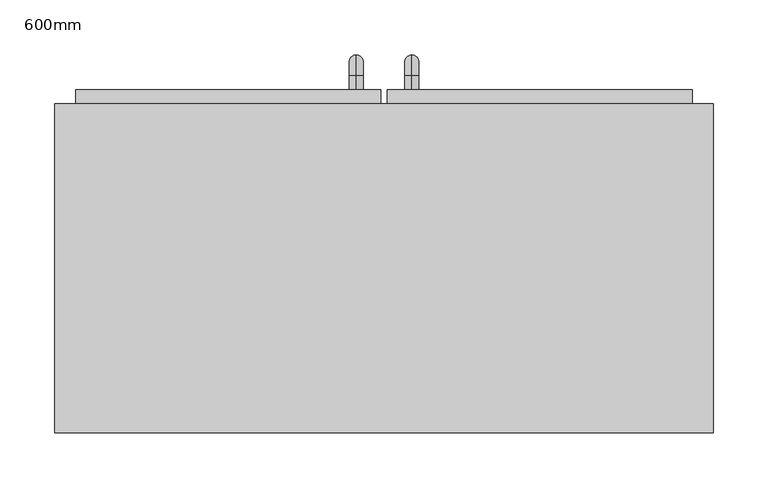
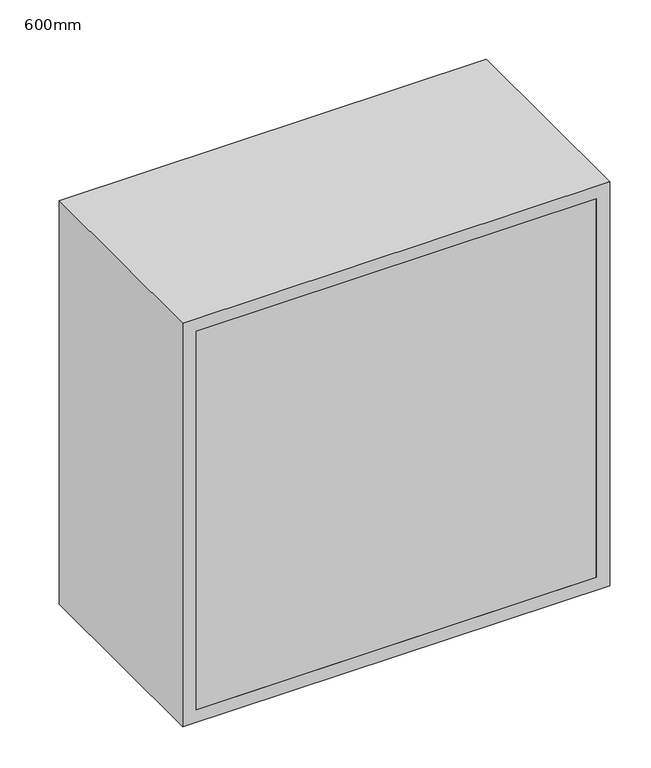
"""IFC4 building model written with IfcOpenShell, lengths in millimetres: furniture geometry, Armário superior-Porta dupla com vidro-Parede : 600mm."""

from ifc_helpers import new_model, si_unit, point, frame, origin, place, context, project, spatial, polyline, circle_curve, ellipse_curve, trimmed, outline, extrude, source, transform, mapped, element, save
from ifc_brep_helpers import plane_surface, cylinder_surface, revolved_surface, advanced_brep


def furniture_600mm_0b7ed25a(model_context):
    return source(origin(), model_context, "Body", "SolidModel", [
        advanced_brep(
        [(55.1711628, 412.7, 1546.05), (55.1711628, 412.7, 1558.75), (55.1711628, 425.4, 1546.05), (55.1711628, 425.4, 1558.75), (55.1711628, 444.45, 1539.7), (55.1711628, 431.75, 1539.7), (55.1711628, 431.75, 1463.5), (55.1711628, 444.45, 1463.5), (55.1711628, 425.4, 1444.45), (55.1711628, 425.4, 1457.15), (55.1711628, 412.7, 1457.15), (55.1711628, 412.7, 1444.45)],
        [
            (0, 1, circle_curve(frame((55.1711628, 412.7, 1552.4), z_axis=(0.0, -1.0, 0.0), x_axis=(0.0, 0.0, -1.0)), 6.35)),
            (1, 0, circle_curve(frame((55.1711628, 412.7, 1552.4), z_axis=(0.0, -1.0, 0.0), x_axis=(0.0, 0.0, -1.0)), 6.35)),
            (0, 2),
            (2, 3, circle_curve(frame((55.1711628, 425.4, 1552.4), z_axis=(0.0, -1.0, 0.0), x_axis=(0.0, 0.0, -1.0)), 6.35)),
            (3, 1),
            (3, 2, circle_curve(frame((55.1711628, 425.4, 1552.4), z_axis=(0.0, -1.0, 0.0), x_axis=(0.0, 0.0, -1.0)), 6.35)),
            (4, 3, circle_curve(frame((55.1711628, 425.4, 1539.7), z_axis=(1.0, 0.0, 0.0), x_axis=(0.0, 0.0, 1.0)), 19.05)),
            (2, 5, circle_curve(frame((55.1711628, 425.4, 1539.7), z_axis=(-1.0, 0.0, 0.0), x_axis=(0.0, 0.0, 1.0)), 6.35)),
            (5, 4, circle_curve(frame((55.1711628, 438.1, 1539.7), z_axis=(0.0, 0.0, 1.0), x_axis=(0.0, -1.0, 0.0)), 6.35)),
            (4, 5, circle_curve(frame((55.1711628, 438.1, 1539.7), z_axis=(0.0, 0.0, 1.0), x_axis=(0.0, -1.0, 0.0)), 6.35)),
            (5, 6),
            (6, 7, circle_curve(frame((55.1711628, 438.1, 1463.5), z_axis=(0.0, 0.0, 1.0), x_axis=(0.0, -1.0, 0.0)), 6.35)),
            (7, 4),
            (7, 6, circle_curve(frame((55.1711628, 438.1, 1463.5), z_axis=(0.0, 0.0, 1.0), x_axis=(0.0, -1.0, 0.0)), 6.35)),
            (8, 7, circle_curve(frame((55.1711628, 425.4, 1463.5), z_axis=(1.0, 0.0, 0.0), x_axis=(0.0, 1.0, 0.0)), 19.05)),
            (6, 9, circle_curve(frame((55.1711628, 425.4, 1463.5), z_axis=(-1.0, 0.0, 0.0), x_axis=(0.0, 1.0, 0.0)), 6.35)),
            (9, 8, circle_curve(frame((55.1711628, 425.4, 1450.8), z_axis=(0.0, 1.0, 0.0), x_axis=(0.0, 0.0, 1.0)), 6.35)),
            (8, 9, circle_curve(frame((55.1711628, 425.4, 1450.8), z_axis=(0.0, 1.0, 0.0), x_axis=(0.0, 0.0, 1.0)), 6.35)),
            (10, 11, circle_curve(frame((55.1711628, 412.7, 1450.8), z_axis=(0.0, -1.0, 0.0), x_axis=(0.0, 0.0, 1.0)), 6.35)),
            (11, 10, circle_curve(frame((55.1711628, 412.7, 1450.8), z_axis=(0.0, -1.0, 0.0), x_axis=(0.0, 0.0, 1.0)), 6.35)),
            (9, 10),
            (11, 8),
        ],
        [
            plane_surface(frame((48.8211628, 412.7, 1552.4), z_axis=(0.0, -1.0, 0.0), x_axis=(0.0, 0.0, 1.0))),
            cylinder_surface(frame((55.1711628, 412.7, 1552.4), z_axis=(0.0, -1.0, 0.0), x_axis=(0.0, 0.0, -1.0)), 6.35),
            revolved_surface(trimmed(ellipse_curve(frame((55.1711628, 425.4, 1552.4), z_axis=(0.0, -1.0, 0.0), x_axis=(0.0, 0.0, -1.0)), 6.35, 6.35), [point((55.1711628, 425.4, 1546.05))], [point((55.1711628, 425.4, 1558.75))], True, "CARTESIAN"), (55.1711628, 425.4, 1539.7), (-1.0, 0.0, 0.0)),
            revolved_surface(trimmed(ellipse_curve(frame((55.1711628, 425.4, 1552.4), z_axis=(0.0, -1.0, 0.0), x_axis=(0.0, 0.0, -1.0)), 6.35, 6.35), [point((55.1711628, 425.4, 1558.75))], [point((55.1711628, 425.4, 1546.05))], True, "CARTESIAN"), (55.1711628, 425.4, 1539.7), (-1.0, 0.0, 0.0)),
            cylinder_surface(frame((55.1711628, 438.1, 1539.7), z_axis=(0.0, 0.0, 1.0), x_axis=(0.0, -1.0, 0.0)), 6.35),
            revolved_surface(trimmed(ellipse_curve(frame((55.1711628, 438.1, 1463.5), z_axis=(0.0, 0.0, 1.0), x_axis=(0.0, -1.0, 0.0)), 6.35, 6.35), [point((55.1711628, 431.75, 1463.5))], [point((55.1711628, 444.45, 1463.5))], True, "CARTESIAN"), (55.1711628, 425.4, 1463.5), (-1.0, 0.0, 0.0)),
            revolved_surface(trimmed(ellipse_curve(frame((55.1711628, 438.1, 1463.5), z_axis=(0.0, 0.0, 1.0), x_axis=(0.0, -1.0, 0.0)), 6.35, 6.35), [point((55.1711628, 444.45, 1463.5))], [point((55.1711628, 431.75, 1463.5))], True, "CARTESIAN"), (55.1711628, 425.4, 1463.5), (-1.0, 0.0, 0.0)),
            plane_surface(frame((48.8211628, 412.7, 1450.8), z_axis=(0.0, -1.0, 0.0), x_axis=(0.0, 0.0, -1.0))),
            cylinder_surface(frame((55.1711628, 425.4, 1450.8), z_axis=(0.0, 1.0, 0.0), x_axis=(0.0, 0.0, 1.0)), 6.35),
        ],
        [
            (0, [[1, 2]]),
            (1, [[-1, 3, 4, 5]]),
            (1, [[-2, -5, 6, -3]]),
            (2, [[7, -4, 8, 9]]),
            (3, [[-8, -6, -7, 10]]),
            (4, [[-9, 11, 12, 13]]),
            (4, [[-10, -13, 14, -11]]),
            (5, [[15, -12, 16, 17]]),
            (6, [[-16, -14, -15, 18]]),
            (7, [[19, 20]]),
            (8, [[-17, 21, -20, 22]]),
            (8, [[-18, -22, -19, -21]]),
        ],
    ),
        advanced_brep(
        [(4.3711628, 412.7, 1546.05), (4.3711628, 412.7, 1558.75), (4.3711628, 425.4, 1546.05), (4.3711628, 425.4, 1558.75), (4.3711628, 444.45, 1539.7), (4.3711628, 431.75, 1539.7), (4.3711628, 431.75, 1463.5), (4.3711628, 444.45, 1463.5), (4.3711628, 425.4, 1444.45), (4.3711628, 425.4, 1457.15), (4.3711628, 412.7, 1457.15), (4.3711628, 412.7, 1444.45)],
        [
            (0, 1, circle_curve(frame((4.3711628, 412.7, 1552.4), z_axis=(0.0, -1.0, 0.0), x_axis=(0.0, 0.0, 1.0)), 6.35)),
            (1, 0, circle_curve(frame((4.3711628, 412.7, 1552.4), z_axis=(0.0, -1.0, 0.0), x_axis=(0.0, 0.0, 1.0)), 6.35)),
            (0, 2),
            (2, 3, circle_curve(frame((4.3711628, 425.4, 1552.4), z_axis=(0.0, -1.0, 0.0), x_axis=(0.0, 0.0, 1.0)), 6.35)),
            (3, 1),
            (3, 2, circle_curve(frame((4.3711628, 425.4, 1552.4), z_axis=(0.0, -1.0, 0.0), x_axis=(0.0, 0.0, 1.0)), 6.35)),
            (4, 3, circle_curve(frame((4.3711628, 425.4, 1539.7), z_axis=(1.0, 0.0, 0.0), x_axis=(0.0, 0.0, 1.0)), 19.05)),
            (2, 5, circle_curve(frame((4.3711628, 425.4, 1539.7), z_axis=(-1.0, 0.0, 0.0), x_axis=(0.0, 0.0, 1.0)), 6.35)),
            (5, 4, circle_curve(frame((4.3711628, 438.1, 1539.7), z_axis=(0.0, 0.0, 1.0), x_axis=(0.0, 1.0, 0.0)), 6.35)),
            (4, 5, circle_curve(frame((4.3711628, 438.1, 1539.7), z_axis=(0.0, 0.0, 1.0), x_axis=(0.0, 1.0, 0.0)), 6.35)),
            (5, 6),
            (6, 7, circle_curve(frame((4.3711628, 438.1, 1463.5), z_axis=(0.0, 0.0, 1.0), x_axis=(0.0, 1.0, 0.0)), 6.35)),
            (7, 4),
            (7, 6, circle_curve(frame((4.3711628, 438.1, 1463.5), z_axis=(0.0, 0.0, 1.0), x_axis=(0.0, 1.0, 0.0)), 6.35)),
            (8, 7, circle_curve(frame((4.3711628, 425.4, 1463.5), z_axis=(1.0, 0.0, 0.0), x_axis=(0.0, 1.0, 0.0)), 19.05)),
            (6, 9, circle_curve(frame((4.3711628, 425.4, 1463.5), z_axis=(-1.0, 0.0, 0.0), x_axis=(0.0, 1.0, 0.0)), 6.35)),
            (9, 8, circle_curve(frame((4.3711628, 425.4, 1450.8), z_axis=(0.0, 1.0, 0.0), x_axis=(0.0, 0.0, -1.0)), 6.35)),
            (8, 9, circle_curve(frame((4.3711628, 425.4, 1450.8), z_axis=(0.0, 1.0, 0.0), x_axis=(0.0, 0.0, -1.0)), 6.35)),
            (10, 11, circle_curve(frame((4.3711628, 412.7, 1450.8), z_axis=(0.0, -1.0, 0.0), x_axis=(0.0, 0.0, -1.0)), 6.35)),
            (11, 10, circle_curve(frame((4.3711628, 412.7, 1450.8), z_axis=(0.0, -1.0, 0.0), x_axis=(0.0, 0.0, -1.0)), 6.35)),
            (9, 10),
            (11, 8),
        ],
        [
            plane_surface(frame((-1.9788372, 412.7, 1552.4), z_axis=(0.0, -1.0, 0.0), x_axis=(0.0, 0.0, 1.0))),
            cylinder_surface(frame((4.3711628, 412.7, 1552.4), z_axis=(0.0, -1.0, 0.0), x_axis=(0.0, 0.0, 1.0)), 6.35),
            revolved_surface(trimmed(ellipse_curve(frame((4.3711628, 425.4, 1552.4), z_axis=(0.0, -1.0, 0.0), x_axis=(0.0, 0.0, 1.0)), 6.35, 6.35), [point((4.3711628, 425.4, 1546.05))], [point((4.3711628, 425.4, 1558.75))], True, "CARTESIAN"), (4.3711628, 425.4, 1539.7), (-1.0, 0.0, 0.0)),
            revolved_surface(trimmed(ellipse_curve(frame((4.3711628, 425.4, 1552.4), z_axis=(0.0, -1.0, 0.0), x_axis=(0.0, 0.0, 1.0)), 6.35, 6.35), [point((4.3711628, 425.4, 1558.75))], [point((4.3711628, 425.4, 1546.05))], True, "CARTESIAN"), (4.3711628, 425.4, 1539.7), (-1.0, 0.0, 0.0)),
            cylinder_surface(frame((4.3711628, 438.1, 1539.7), z_axis=(0.0, 0.0, 1.0), x_axis=(0.0, 1.0, 0.0)), 6.35),
            revolved_surface(trimmed(ellipse_curve(frame((4.3711628, 438.1, 1463.5), z_axis=(0.0, 0.0, 1.0), x_axis=(0.0, 1.0, 0.0)), 6.35, 6.35), [point((4.3711628, 431.75, 1463.5))], [point((4.3711628, 444.45, 1463.5))], True, "CARTESIAN"), (4.3711628, 425.4, 1463.5), (-1.0, 0.0, 0.0)),
            revolved_surface(trimmed(ellipse_curve(frame((4.3711628, 438.1, 1463.5), z_axis=(0.0, 0.0, 1.0), x_axis=(0.0, 1.0, 0.0)), 6.35, 6.35), [point((4.3711628, 444.45, 1463.5))], [point((4.3711628, 431.75, 1463.5))], True, "CARTESIAN"), (4.3711628, 425.4, 1463.5), (-1.0, 0.0, 0.0)),
            plane_surface(frame((-1.9788372, 412.7, 1450.8), z_axis=(0.0, -1.0, 0.0), x_axis=(0.0, 0.0, -1.0))),
            cylinder_surface(frame((4.3711628, 425.4, 1450.8), z_axis=(0.0, 1.0, 0.0), x_axis=(0.0, 0.0, -1.0)), 6.35),
        ],
        [
            (0, [[1, 2]]),
            (1, [[-1, 3, 4, 5]]),
            (1, [[-2, -5, 6, -3]]),
            (2, [[7, -4, 8, 9]]),
            (3, [[-8, -6, -7, 10]]),
            (4, [[-9, 11, 12, 13]]),
            (4, [[-10, -13, 14, -11]]),
            (5, [[15, -12, 16, 17]]),
            (6, [[-16, -14, -15, 18]]),
            (7, [[19, 20]]),
            (8, [[-17, 21, -20, 22]]),
            (8, [[-18, -22, -19, -21]]),
        ],
    ),
        extrude(outline(polyline([(64.6961628, 393.65), (278.9711628, 393.65), (278.9711628, 387.3), (64.6961628, 387.3), (64.6961628, 393.65)])), frame((0.0, 0.0, 1450.8), z_axis=(0.0, 0.0, 1.0), x_axis=(1.0, 0.0, 0.0)), (0.0, 0.0, 1.0), 498.4),
        extrude(outline(polyline([(-219.4288372, 393.65), (-5.1538372, 393.65), (-5.1538372, 387.3), (-219.4288372, 387.3), (-219.4288372, 393.65)])), frame((0.0, 0.0, 1450.8), z_axis=(0.0, 0.0, 1.0), x_axis=(1.0, 0.0, 0.0)), (0.0, 0.0, 1.0), 498.4),
        extrude(outline(polyline([(1980.95, 32.9461628), (1419.05, 32.9461628), (1419.05, 310.7211628), (1980.95, 310.7211628), (1980.95, 32.9461628)]), holes=[polyline([(1450.8, 64.6961628), (1949.2, 64.6961628), (1949.2, 278.9711628), (1450.8, 278.9711628), (1450.8, 64.6961628)])]), frame((0.0, 380.95, 0.0), z_axis=(0.0, 1.0, 0.0), x_axis=(0.0, 0.0, 1.0)), (0.0, 0.0, 1.0), 31.75),
        extrude(outline(polyline([(1419.05, -251.1788372), (1419.05, 26.5961628), (1980.95, 26.5961628), (1980.95, -251.1788372), (1419.05, -251.1788372)]), holes=[polyline([(1949.2, -5.1538372), (1450.8, -5.1538372), (1450.8, -219.4288372), (1949.2, -219.4288372), (1949.2, -5.1538372)])]), frame((0.0, 380.95, 0.0), z_axis=(0.0, 1.0, 0.0), x_axis=(0.0, 0.0, 1.0)), (0.0, 0.0, 1.0), 31.75),
        extrude(outline(polyline([(310.7211628, 100.0), (-251.1788372, 100.0), (-251.1788372, 119.05), (310.7211628, 119.05), (310.7211628, 100.0)])), frame((0.0, 0.0, 1419.05), z_axis=(0.0, 0.0, 1.0), x_axis=(1.0, 0.0, 0.0)), (0.0, 0.0, 1.0), 561.9),
        extrude(outline(polyline([(2000.0, -270.2288372), (1400.0, -270.2288372), (1400.0, 329.7711628), (2000.0, 329.7711628), (2000.0, -270.2288372)]), holes=[polyline([(1980.95, -251.1788372), (1980.95, 310.7211628), (1419.05, 310.7211628), (1419.05, -251.1788372), (1980.95, -251.1788372)])]), frame((0.0, 100.0, 0.0), z_axis=(0.0, 1.0, 0.0), x_axis=(0.0, 0.0, 1.0)), (0.0, 0.0, 1.0), 300.0),
    ])


if __name__ == "__main__":
    model = new_model("IFC4")
    model_context = context("Model", 3, world=origin())
    ifc_project = project(units=[si_unit("LENGTHUNIT", "METRE", prefix="MILLI")], contexts=[model_context])
    site = spatial("IfcSite", under=ifc_project)
    building = spatial("IfcBuilding", under=site)
    placement = place(None, origin())
    furniture_600mm_shape = furniture_600mm_0b7ed25a(model_context)
    element("IfcFurniture", 1, ObjectType="Armário superior-Porta dupla com vidro-Parede : 600mm", at=placement, inside=building, context=model_context, shape_type="MappedRepresentation", body=[
        mapped(furniture_600mm_shape, transform((0.0, 0.0, 0.0), x_axis=(1.0, 0.0, 0.0), y_axis=(0.0, 1.0, 0.0), z_axis=(0.0, 0.0, 1.0))),
    ])
    save(model, "model.ifc")

# Revit data of these elements
# Project information
#   Data de emissão do projeto = "Data de emissão"
#   Status do projeto = "Status do projeto"
#   Nome do cliente = "Proprietário"
#   Endereço do projeto = "Insira aqui o endereço"
#   Nome do projeto = "Nome do projeto"
#   Número do projeto = "0001"
# Type "Armário superior-Porta dupla com vidro-Parede : 600mm"
#   Depth = 300 mm
#   Height = 600 mm
#   Topo do armário = 2000 mm
#   Width = 600 mm
#   Material do armário = none
#   Material da porta/gaveta = none
#   Material do puxador = Armários - Puxadores
#   Material do painel = Armários - Painel/Vidro
# Element 1 (IfcFurniture, "Armário superior-Porta dupla com vidro-Parede : 600mm")
#   Materials on its faces: "Armários", "Armários - Puxadores", "Armários - Painel/Vidro"
# Materials
#   "Armários - Puxadores": class "Metal", colour RGB 57 57 57, transparency 0
#   "Armários - Painel/Vidro": class "Diversos", colour RGB 252 255 255, transparency 0.72
#   "Armários": class "Diversos", colour RGB 249 249 249, transparency 0
